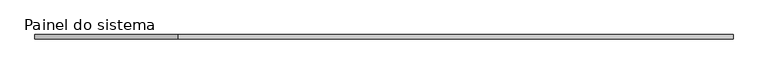
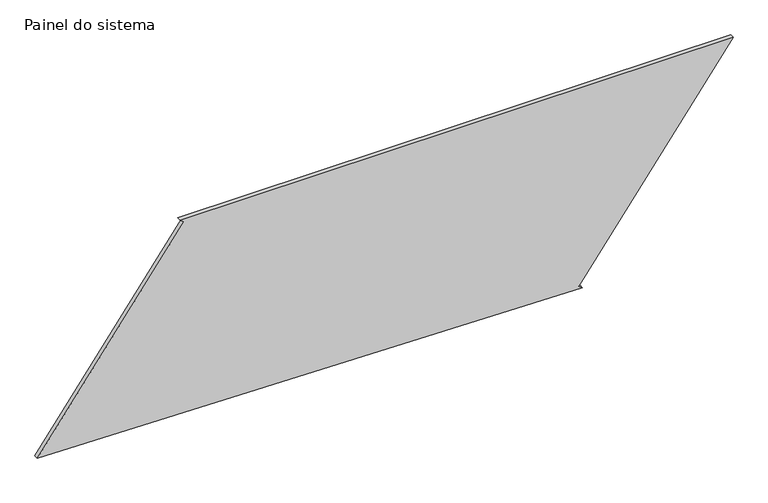
"""IFC4 building model written with IfcOpenShell, lengths in millimetres: plate geometry, Painel do sistema : Envidraçado."""

from ifc_helpers import new_model, si_unit, frame, origin, place, context, project, spatial, polyline, outline, extrude, source, transform, mapped, element, save


def painel_do_sistema_9f354deb(model_context):
    return source(origin(), model_context, "Body", "SweptSolid", [
        extrude(outline(polyline([(0.0, 1129.3962645), (14.8374505, 1109.2753783), (1212.3202898, 1992.3176123), (1212.3202898, -1173.085874), (1197.4828393, -1152.9649878), (59.2469484, -1992.3176123), (0.0, 1129.3962645)])), frame((0.0, 24.5, 0.0), z_axis=(0.0, 1.0, 0.0), x_axis=(0.0, 0.0, 1.0)), (0.0, 0.0, 1.0), 25.0),
    ])


if __name__ == "__main__":
    model = new_model("IFC4")
    model_context = context("Model", 3, world=origin())
    ifc_project = project(units=[si_unit("LENGTHUNIT", "METRE", prefix="MILLI")], contexts=[model_context])
    site = spatial("IfcSite", under=ifc_project)
    building = spatial("IfcBuilding", under=site)
    placement = place(None, origin())
    painel_do_sistema_shape = painel_do_sistema_9f354deb(model_context)
    element("IfcPlate", 1, ObjectType="Painel do sistema : Envidraçado", at=placement, inside=building, context=model_context, shape_type="MappedRepresentation", body=[
        mapped(painel_do_sistema_shape, transform((0.0, 0.0, 0.0), x_axis=(1.0, 0.0, 0.0), y_axis=(0.0, 1.0, 0.0), z_axis=(0.0, 0.0, 1.0))),
    ])
    save(model, "model.ifc")

# Revit data of these elements
# Type "Painel do sistema : Envidraçado"
#   Construction Type Id = "GSP4R"
#   Analytic Construction = "Vidraça única Pilkington 1/8 pol"
#   Visual Light Transmittance = 0.9
#   Solar Heat Gain Coefficient = 0.86
#   Heat Transfer Coefficient (U) = 6.7069 W/(m²·K)
# Element 1 (IfcPlate, "Painel do sistema : Envidraçado")
#   Materials on its faces: "Vidro"
# Materials
#   "Vidro": class "Vidro", colour RGB 0 128 192, transparency 0.9, Description = "Vidro de sílica", Cost = 0
